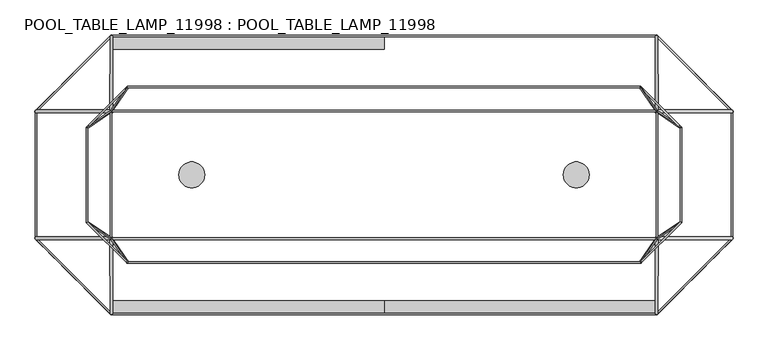
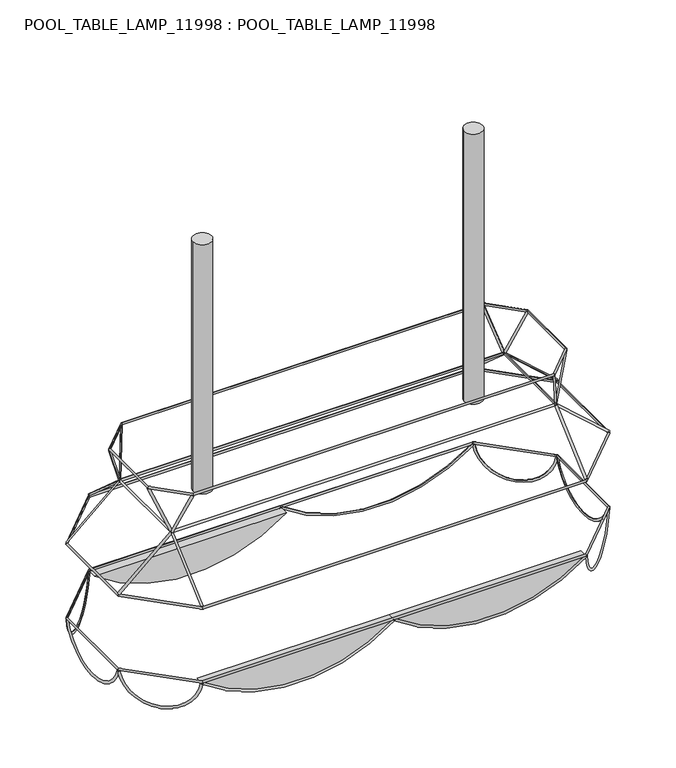
"""IFC4 building model written with IfcOpenShell, lengths in millimetres: proxy geometry, POOL_TABLE_LAMP_11998 : POOL_TABLE_LAMP_11998."""

from ifc_helpers import new_model, si_unit, point, frame, frame_2d, origin, origin_2d, place, context, project, spatial, polyline, circle_curve, ellipse_curve, trimmed, segment, composite_curve, outline, extrude, source, transform, mapped, element, save
from ifc_brep_helpers import plane_surface, cylinder_surface, revolved_surface, advanced_brep


def pool_table_lamp_11998_pool_table_lamp_11998_82cd1bbc(model_context):
    return source(origin(), model_context, "Body", "SolidModel", [
        extrude(outline(composite_curve([segment(trimmed(circle_curve(frame_2d((-308.8341807, 246.5034627)), 25.4), [point((-283.4341807, 246.5034627))], [point((-334.2341807, 246.5034627))], False, "CARTESIAN"), True, "CONTINUOUS"), segment(trimmed(circle_curve(frame_2d((-308.8341807, 246.5034627)), 25.4), [point((-334.2341807, 246.5034627))], [point((-283.4341807, 246.5034627))], False, "CARTESIAN"), True, "CONTINUOUS")], self_intersect=False)), frame((0.0, 0.0, 2030.2376392), z_axis=(0.0, 0.0, 1.0), x_axis=(1.0, 0.0, 0.0)), (0.0, 0.0, 1.0), 792.7919161),
        extrude(outline(composite_curve([segment(trimmed(circle_curve(frame_2d((-1061.7579936, 246.5034627)), 25.4), [point((-1087.1579936, 246.5034627))], [point((-1036.3579936, 246.5034627))], False, "CARTESIAN"), True, "CONTINUOUS"), segment(trimmed(circle_curve(frame_2d((-1061.7579936, 246.5034627)), 25.4), [point((-1036.3579936, 246.5034627))], [point((-1087.1579936, 246.5034627))], False, "CARTESIAN"), True, "CONTINUOUS")], self_intersect=False)), frame((0.0, 0.0, 2030.2376392), z_axis=(0.0, 0.0, 1.0), x_axis=(1.0, 0.0, 0.0)), (0.0, 0.0, 1.0), 731.5822221),
        extrude(outline(composite_curve([segment(polyline([(0.0, -3.175), (0.0, 3.175)]), True, "CONTINUOUS"), segment(trimmed(circle_curve(origin_2d(), 3.175), [point((0.0, 3.175))], [point((0.0, -3.175))], False, "CARTESIAN"), True, "CONTINUOUS")], self_intersect=False)), frame((-1218.1975115, 370.1790475, 2030.2376392), z_axis=(-0.3368565795297006, -0.2287745741588877, 0.9133399361935128), x_axis=(-0.7046441830524278, 0.7046441830524578, -0.08338555378907853)), (0.0, 0.0, 1.0), 138.9524053),
        extrude(outline(composite_curve([segment(polyline([(0.0, -3.175), (0.0, 3.1750001)]), True, "CONTINUOUS"), segment(trimmed(circle_curve(origin_2d(), 3.175), [point((0.0, 3.1750001))], [point((0.0, -3.175))], False, "CARTESIAN"), True, "CONTINUOUS")], self_intersect=False)), frame((-1218.1975115, 122.827878, 2030.2376392), z_axis=(-0.33685657952969905, 0.22877457415888985, 0.9133399361935128), x_axis=(-0.7046441830524323, -0.7046441830524531, -0.08338555378907848)), (0.0, 0.0, 1.0), 138.9524053),
        extrude(outline(composite_curve([segment(polyline([(0.0, -3.1750001), (0.0, 3.175)]), True, "CONTINUOUS"), segment(trimmed(circle_curve(origin_2d(), 3.175), [point((0.0, 3.175))], [point((0.0, -3.1750001))], False, "CARTESIAN"), True, "CONTINUOUS")], self_intersect=False)), frame((-152.3946628, 122.827878, 2030.2376392), z_axis=(0.33685657952969905, 0.22877457415888985, 0.9133399361935128), x_axis=(0.7046441830524323, -0.7046441830524531, -0.08338555378907847)), (0.0, 0.0, 1.0), 138.9524053),
        extrude(outline(composite_curve([segment(polyline([(0.0, -3.175), (0.0, 3.175)]), True, "CONTINUOUS"), segment(trimmed(circle_curve(origin_2d(), 3.175), [point((0.0, 3.175))], [point((0.0, -3.175))], False, "CARTESIAN"), True, "CONTINUOUS")], self_intersect=False)), frame((-152.3946628, 370.1790475, 2030.2376392), z_axis=(0.33685657952969744, -0.22877457415889219, 0.9133399361935128), x_axis=(0.704644183052437, 0.7046441830524486, -0.08338555378907836)), (0.0, 0.0, 1.0), 138.9524053),
        extrude(outline(composite_curve([segment(polyline([(0.0, -3.1749999), (0.0, 3.175)]), True, "CONTINUOUS"), segment(trimmed(circle_curve(origin_2d(), 3.175), [point((0.0, 3.175))], [point((0.0, -3.1749999))], False, "CARTESIAN"), True, "CONTINUOUS")], self_intersect=False)), frame((-152.2155087, 369.9998934, 2030.2376392), z_axis=(-0.22877457415889185, 0.33685657952969766, 0.9133399361935128), x_axis=(0.7046441830524492, 0.7046441830524363, -0.0833855537890783)), (0.0, 0.0, 1.0), 138.9524053),
        extrude(outline(composite_curve([segment(polyline([(0.0, -3.175), (0.0, 3.175)]), True, "CONTINUOUS"), segment(trimmed(circle_curve(origin_2d(), 3.175), [point((0.0, 3.175))], [point((0.0, -3.175))], False, "CARTESIAN"), True, "CONTINUOUS")], self_intersect=False)), frame((-152.2155087, 123.007032, 2030.2376392), z_axis=(-0.22877457415889405, -0.3368565795296962, 0.9133399361935128), x_axis=(0.7046441830524446, -0.704644183052441, -0.08338555378907837)), (0.0, 0.0, 1.0), 138.9524053),
        extrude(outline(composite_curve([segment(polyline([(0.0, -3.1750001), (0.0, 3.175)]), True, "CONTINUOUS"), segment(trimmed(circle_curve(origin_2d(), 3.175), [point((0.0, 3.175))], [point((0.0, -3.1750001))], False, "CARTESIAN"), True, "CONTINUOUS")], self_intersect=False)), frame((-1218.3766655, 123.007032, 2030.2376392), z_axis=(0.22877457415889405, -0.3368565795296962, 0.9133399361935128), x_axis=(-0.7046441830524446, -0.704644183052441, -0.08338555378907837)), (0.0, 0.0, 1.0), 138.9524053),
        extrude(outline(composite_curve([segment(polyline([(0.0, -3.175), (1e-07, 3.175)]), True, "CONTINUOUS"), segment(trimmed(circle_curve(origin_2d(), 3.175), [point((1e-07, 3.175))], [point((0.0, -3.175))], False, "CARTESIAN"), True, "CONTINUOUS")], self_intersect=False)), frame((-1218.3766655, 369.9998934, 2030.2376392), z_axis=(0.22877457415889615, 0.33685657952969483, 0.9133399361935128), x_axis=(-0.70464418305244, 0.7046441830524455, -0.0833855537890785)), (0.0, 0.0, 1.0), 138.9524053),
        advanced_brep(
        [(-105.6341807, 338.43682, 2162.175), (-184.0042861, 416.8069254, 2162.175), (-184.0042861, 416.8069254, 2155.825), (-105.6341807, 338.43682, 2155.825), (-1186.5878882, 416.8069254, 2162.175), (-1186.5878882, 416.8069254, 2155.825), (-1264.9579936, 338.43682, 2162.175), (-1264.9579936, 338.43682, 2155.825), (-1264.9579936, 154.5701054, 2162.175), (-1264.9579936, 154.5701054, 2155.825), (-1186.5878882, 76.2, 2162.175), (-1186.5878882, 76.2, 2155.825), (-184.0042861, 76.2, 2162.175), (-184.0042861, 76.2, 2155.825), (-105.6341807, 154.5701054, 2162.175), (-105.6341807, 154.5701054, 2155.825)],
        [
            (0, 1),
            (1, 2),
            (2, 3),
            (3, 0),
            (0, 3, ellipse_curve(frame((-105.6341807, 338.43682, 2159.0), z_axis=(-0.38268343236509084, 0.9238795325112865, 0.0), x_axis=(0.923879532511286, 0.38268343236509184, 0.0)), 3.4365952, 3.175)),
            (2, 1, ellipse_curve(frame((-184.0042861, 416.8069254, 2159.0), z_axis=(0.9238795325112863, -0.382683432365091, 0.0), x_axis=(-0.3826834323650911, -0.9238795325112862, 0.0)), 3.4365952, 3.175)),
            (1, 4),
            (4, 5),
            (5, 2),
            (5, 4, ellipse_curve(frame((-1186.5878882, 416.8069254, 2159.0), z_axis=(0.9238795325112887, 0.38268343236508495, 0.0), x_axis=(0.38268343236508523, -0.9238795325112888, 0.0)), 3.4365952, 3.175)),
            (4, 6),
            (6, 7),
            (7, 5),
            (7, 6, ellipse_curve(frame((-1264.9579936, 338.43682, 2159.0), z_axis=(0.38268343236509156, 0.9238795325112859, 0.0), x_axis=(0.9238795325112862, -0.3826834323650906, 0.0)), 3.4365952, 3.175)),
            (6, 8),
            (8, 9),
            (9, 7),
            (9, 8, ellipse_curve(frame((-1264.9579936, 154.5701054, 2159.0), z_axis=(-0.38268343236508867, 0.9238795325112872, 0.0), x_axis=(0.9238795325112872, 0.38268343236508895, 0.0)), 3.4365952, 3.175)),
            (8, 10),
            (10, 11),
            (11, 9),
            (11, 10, ellipse_curve(frame((-1186.5878882, 76.2, 2159.0), z_axis=(-0.9238795325112863, 0.38268343236509084, 0.0), x_axis=(0.38268343236509084, 0.9238795325112864, 0.0)), 3.4365952, 3.175)),
            (10, 12),
            (12, 13),
            (13, 11),
            (13, 12, ellipse_curve(frame((-184.0042861, 76.2, 2159.0), z_axis=(-0.9238795325112887, -0.38268343236508484, 0.0), x_axis=(-0.3826834323650852, 0.9238795325112886, 0.0)), 3.4365952, 3.175)),
            (12, 14),
            (14, 15),
            (15, 13),
            (15, 14, ellipse_curve(frame((-105.6341807, 154.5701054, 2159.0), z_axis=(-0.38268343236509555, -0.9238795325112844, 0.0), x_axis=(-0.9238795325112842, 0.38268343236509583, 0.0)), 3.4365952, 3.175)),
            (14, 0),
            (3, 15),
        ],
        [
            plane_surface(frame((-105.6341807, 338.43682, 2159.0), z_axis=(-0.7071067811865449, -0.7071067811865501, 0.0), x_axis=(-0.7071067811865501, 0.7071067811865449, 0.0))),
            cylinder_surface(frame((-105.6341807, 338.43682, 2159.0), z_axis=(0.7071067811865503, -0.7071067811865448, 0.0), x_axis=(-0.7071067811865448, -0.7071067811865503, 0.0)), 3.175),
            plane_surface(frame((-184.0042861, 416.8069254, 2159.0), z_axis=(0.0, -1.0, 0.0), x_axis=(-1.0, 0.0, 0.0))),
            cylinder_surface(frame((-184.0042861, 416.8069254, 2159.0), z_axis=(1.0, 0.0, 0.0), x_axis=(0.0, -1.0, 0.0)), 3.175),
            plane_surface(frame((-1186.5878882, 416.8069254, 2159.0), z_axis=(0.7071067811865451, -0.70710678118655, 0.0), x_axis=(-0.70710678118655, -0.7071067811865451, 0.0))),
            cylinder_surface(frame((-1186.5878882, 416.8069254, 2159.0), z_axis=(0.7071067811865503, 0.7071067811865448, 0.0), x_axis=(0.7071067811865448, -0.7071067811865503, 0.0)), 3.175),
            plane_surface(frame((-1264.9579936, 338.43682, 2159.0), z_axis=(1.0, 0.0, 0.0), x_axis=(0.0, -1.0, 0.0))),
            cylinder_surface(frame((-1264.9579936, 338.43682, 2159.0), z_axis=(0.0, 1.0, 0.0), x_axis=(1.0, 0.0, 0.0)), 3.175),
            plane_surface(frame((-1264.9579936, 154.5701054, 2159.0), z_axis=(0.7071067811865496, 0.7071067811865456, 0.0), x_axis=(0.7071067811865456, -0.7071067811865496, 0.0))),
            cylinder_surface(frame((-1264.9579936, 154.5701054, 2159.0), z_axis=(-0.7071067811865459, 0.7071067811865491, 0.0), x_axis=(0.7071067811865491, 0.7071067811865459, 0.0)), 3.175),
            plane_surface(frame((-1186.5878882, 76.2, 2159.0), z_axis=(0.0, 1.0, 0.0), x_axis=(1.0, 0.0, 0.0))),
            cylinder_surface(frame((-1186.5878882, 76.2, 2159.0), z_axis=(-1.0, 0.0, 0.0), x_axis=(0.0, 1.0, 0.0)), 3.175),
            plane_surface(frame((-184.0042861, 76.2, 2159.0), z_axis=(-0.70710678118654, 0.7071067811865551, 0.0), x_axis=(0.7071067811865551, 0.70710678118654, 0.0))),
            cylinder_surface(frame((-184.0042861, 76.2, 2159.0), z_axis=(-0.7071067811865551, -0.70710678118654, 0.0), x_axis=(-0.70710678118654, 0.7071067811865551, 0.0)), 3.175),
            plane_surface(frame((-105.6341807, 154.5701054, 2159.0), z_axis=(-1.0, 0.0, 0.0), x_axis=(0.0, 1.0, 0.0))),
            cylinder_surface(frame((-105.6341807, 154.5701054, 2159.0), z_axis=(0.0, -1.0, 0.0), x_axis=(-1.0, 0.0, 0.0)), 3.175),
        ],
        [
            (0, [[1, 2, 3, 4]]),
            (1, [[5, -3, 6, -1]]),
            (2, [[-2, 7, 8, 9]]),
            (3, [[-6, -9, 10, -7]]),
            (4, [[-8, 11, 12, 13]]),
            (5, [[-10, -13, 14, -11]]),
            (6, [[-12, 15, 16, 17]]),
            (7, [[-14, -17, 18, -15]]),
            (8, [[-16, 19, 20, 21]]),
            (9, [[-18, -21, 22, -19]]),
            (10, [[-20, 23, 24, 25]]),
            (11, [[-22, -25, 26, -23]]),
            (12, [[-24, 27, 28, 29]]),
            (13, [[-26, -29, 30, -27]]),
            (14, [[-28, 31, -4, 32]]),
            (15, [[-30, -32, -5, -31]]),
        ],
    ),
        advanced_brep(
        [(-1218.3766655, 123.007032, 2028.825), (-1218.3766655, 123.007032, 2035.175), (-1218.3766655, 369.9998934, 2035.175), (-1218.3766655, 369.9998934, 2028.825), (-152.2155087, 369.9998934, 2035.175), (-152.2155087, 369.9998934, 2028.825), (-152.2155087, 123.007032, 2035.175), (-152.2155087, 123.007032, 2028.825)],
        [
            (0, 1, ellipse_curve(frame((-1218.3766655, 123.007032, 2032.0), z_axis=(-0.707106781186548, 0.707106781186547, 0.0), x_axis=(-0.707106781186547, -0.7071067811865479, 0.0)), 4.4901281, 3.175)),
            (1, 2),
            (2, 3, ellipse_curve(frame((-1218.3766655, 369.9998934, 2032.0), z_axis=(-0.7071067811865492, -0.7071067811865457, 0.0), x_axis=(0.7071067811865456, -0.7071067811865493, 0.0)), 4.4901281, 3.175)),
            (3, 0),
            (3, 2),
            (1, 0),
            (2, 4),
            (4, 5, ellipse_curve(frame((-152.2155087, 369.9998934, 2032.0), z_axis=(-0.7071067811865446, 0.7071067811865506, 0.0), x_axis=(-0.7071067811865505, -0.7071067811865446, 0.0)), 4.4901281, 3.175)),
            (5, 3),
            (5, 4),
            (4, 6),
            (6, 7, ellipse_curve(frame((-152.2155087, 123.007032, 2032.0), z_axis=(0.7071067811865482, 0.7071067811865468, 0.0), x_axis=(-0.7071067811865468, 0.7071067811865482, 0.0)), 4.4901281, 3.175)),
            (7, 5),
            (7, 6),
            (6, 1),
            (0, 7),
        ],
        [
            cylinder_surface(frame((-1218.3766655, 123.007032, 2032.0), z_axis=(0.0, -1.0, 0.0), x_axis=(-1.0, 0.0, 0.0)), 3.175),
            plane_surface(frame((-1218.3766655, 123.007032, 2032.0), z_axis=(1.0, 0.0, 0.0), x_axis=(0.0, 1.0, 0.0))),
            cylinder_surface(frame((-1218.3766655, 369.9998934, 2032.0), z_axis=(-1.0, 0.0, 0.0), x_axis=(0.0, 1.0, 0.0)), 3.175),
            plane_surface(frame((-1218.3766655, 369.9998934, 2032.0), z_axis=(0.0, -1.0, 0.0), x_axis=(1.0, 0.0, 0.0))),
            cylinder_surface(frame((-152.2155087, 369.9998934, 2032.0), z_axis=(0.0, 1.0, 0.0), x_axis=(1.0, 0.0, 0.0)), 3.175),
            plane_surface(frame((-152.2155087, 369.9998934, 2032.0), z_axis=(-1.0, 0.0, 0.0), x_axis=(0.0, -1.0, 0.0))),
            cylinder_surface(frame((-152.2155087, 123.007032, 2032.0), z_axis=(1.0, 0.0, 0.0), x_axis=(0.0, -1.0, 0.0)), 3.175),
            plane_surface(frame((-152.2155087, 123.007032, 2032.0), z_axis=(0.0, 1.0, 0.0), x_axis=(-1.0, 0.0, 0.0))),
        ],
        [
            (0, [[1, 2, 3, 4]]),
            (1, [[-4, 5, -2, 6]]),
            (2, [[-3, 7, 8, 9]]),
            (3, [[-5, -9, 10, -7]]),
            (4, [[-8, 11, 12, 13]]),
            (5, [[-10, -13, 14, -11]]),
            (6, [[-12, 15, -1, 16]]),
            (7, [[-14, -16, -6, -15]]),
        ],
    ),
        advanced_brep(
        [(-1365.4872204, 366.9890164, 1677.4075935), (-1365.4872204, 373.0107705, 1675.3924065), (-1365.4872204, 119.996155, 1675.3924065), (-1365.4872204, 126.017909, 1677.4075935)],
        [
            (0, 1),
            (1, 0, circle_curve(frame((-1365.4872204, 369.9998934, 1676.4), z_axis=(0.0, 0.3173522867463232, 0.9483077169868858), x_axis=(0.0, 0.9483077169868858, -0.3173522867463232)), 3.175)),
            (2, 3),
            (3, 2, circle_curve(frame((-1365.4872204, 123.007032, 1676.4), z_axis=(0.0, -0.3173522867463063, 0.9483077169868914), x_axis=(0.0, -0.9483077169868914, -0.3173522867463063)), 3.175)),
            (3, 0, circle_curve(frame((-1365.4872204, 246.5034627, 1717.728225), z_axis=(1.0, 0.0, 0.0), x_axis=(0.0, 0.9483077169868859, -0.317352286746323)), 127.053225)),
            (1, 2, circle_curve(frame((-1365.4872204, 246.5034627, 1717.728225), z_axis=(-1.0, 0.0, 0.0), x_axis=(0.0, 0.9483077169868859, -0.317352286746323)), 133.403225)),
        ],
        [
            plane_surface(frame((-1365.4872204, 369.9998934, 1676.4), z_axis=(0.0, 0.317352286746323, 0.9483077169868859), x_axis=(-1.0, 0.0, 0.0))),
            plane_surface(frame((-1365.4872204, 123.007032, 1676.4), z_axis=(0.0, -0.31735228674630656, 0.9483077169868913), x_axis=(-1.0, 0.0, 0.0))),
            revolved_surface(trimmed(ellipse_curve(frame((-1365.4872204, 369.9998934, 1676.4), z_axis=(0.0, 0.3173522867463232, 0.9483077169868858), x_axis=(0.0, 0.9483077169868858, -0.3173522867463232)), 3.175, 3.175), [point((-1365.4872204, 373.0107705, 1675.3924065))], [point((-1365.4872204, 366.9890164, 1677.4075935))], True, "CARTESIAN"), (-1365.4872204, 246.5034627, 1717.728225), (-1.0, 0.0, 0.0)),
            plane_surface(frame((-1365.4872204, 246.5034627, 1717.728225), z_axis=(1.0, 0.0, 0.0), x_axis=(0.0, 0.9483077169868859, -0.317352286746323))),
        ],
        [
            (0, [[1, 2]]),
            (1, [[3, 4]]),
            (2, [[5, -2, 6, -4]]),
            (3, [[-6, -1, -5, -3]]),
        ],
    ),
        advanced_brep(
        [(-5.1049539, 373.0107705, 1675.3924065), (-5.1049539, 366.9890164, 1677.4075935), (-5.1049539, 126.017909, 1677.4075935), (-5.1049539, 119.996155, 1675.3924065)],
        [
            (0, 1),
            (1, 0, circle_curve(frame((-5.1049539, 369.9998934, 1676.4), z_axis=(0.0, 0.3173522867463232, 0.9483077169868858), x_axis=(0.0, 0.9483077169868858, -0.3173522867463232)), 3.175)),
            (2, 3),
            (3, 2, circle_curve(frame((-5.1049539, 123.007032, 1676.4), z_axis=(0.0, -0.3173522867463063, 0.9483077169868914), x_axis=(0.0, -0.9483077169868914, -0.3173522867463063)), 3.175)),
            (3, 0, circle_curve(frame((-5.1049539, 246.5034627, 1717.728225), z_axis=(1.0, 0.0, 0.0), x_axis=(0.0, 0.9483077169868859, -0.317352286746323)), 133.403225)),
            (1, 2, circle_curve(frame((-5.1049539, 246.5034627, 1717.728225), z_axis=(-1.0, 0.0, 0.0), x_axis=(0.0, 0.9483077169868859, -0.317352286746323)), 127.053225)),
        ],
        [
            plane_surface(frame((-5.1049539, 369.9998934, 1676.4), z_axis=(0.0, 0.317352286746323, 0.9483077169868859), x_axis=(1.0, 0.0, 0.0))),
            plane_surface(frame((-5.1049539, 123.007032, 1676.4), z_axis=(0.0, -0.31735228674630656, 0.9483077169868913), x_axis=(1.0, 0.0, 0.0))),
            revolved_surface(trimmed(ellipse_curve(frame((-5.1049539, 369.9998934, 1676.4), z_axis=(0.0, 0.3173522867463232, 0.9483077169868858), x_axis=(0.0, 0.9483077169868858, -0.3173522867463232)), 3.175, 3.175), [point((-5.1049539, 366.9890164, 1677.4075935))], [point((-5.1049539, 373.0107705, 1675.3924065))], True, "CARTESIAN"), (-5.1049539, 246.5034627, 1717.728225), (-1.0, 0.0, 0.0)),
            plane_surface(frame((-5.1049539, 246.5034627, 1717.728225), z_axis=(-1.0, 0.0, 0.0), x_axis=(0.0, 0.9483077169868859, -0.317352286746323))),
        ],
        [
            (0, [[1, 2]]),
            (1, [[3, 4]]),
            (2, [[5, -2, 6, -4]]),
            (3, [[-6, -1, -5, -3]]),
        ],
    ),
        advanced_brep(
        [(-1363.4950625, 120.7891702, 1676.8927506), (-1367.9307861, 125.2248938, 1675.9072494), (-1216.4782253, -26.227667, 1675.9072494), (-1220.9139489, -21.7919434, 1676.8927506)],
        [
            (0, 1),
            (1, 0, circle_curve(frame((-1365.7129243, 123.007032, 1676.4), z_axis=(-0.10974087344321956, 0.1097408734432232, 0.9878835363502307), x_axis=(-0.6985391475757914, 0.6985391475757993, -0.15519703157007309)), 3.175)),
            (2, 3),
            (3, 2, circle_curve(frame((-1218.6960871, -24.0098052, 1676.4), z_axis=(0.10974087344321433, -0.10974087344321463, 0.9878835363502323), x_axis=(0.6985391475757923, -0.6985391475758007, -0.1551970315700634)), 3.175)),
            (3, 0, circle_curve(frame((-1292.2045057, 49.4986134, 1692.7316378), z_axis=(0.7071067811865517, 0.7071067811865435, 0.0), x_axis=(-0.6985391475757914, 0.6985391475757993, -0.1551970315700732)), 102.0566378)),
            (1, 2, circle_curve(frame((-1292.2045057, 49.4986134, 1692.7316378), z_axis=(-0.7071067811865517, -0.7071067811865435, 0.0), x_axis=(-0.6985391475757914, 0.6985391475757993, -0.1551970315700732)), 108.4066378)),
        ],
        [
            plane_surface(frame((-1365.7129243, 123.007032, 1676.4), z_axis=(-0.10974087344321996, 0.10974087344322306, 0.987883536350231), x_axis=(-0.7071067811865518, -0.7071067811865435, 0.0))),
            plane_surface(frame((-1218.6960871, -24.0098052, 1676.4), z_axis=(0.10974087344321468, -0.10974087344321405, 0.9878835363502325), x_axis=(-0.7071067811865517, -0.7071067811865436, 0.0))),
            revolved_surface(trimmed(ellipse_curve(frame((-1365.7129243, 123.007032, 1676.4), z_axis=(-0.10974087344321956, 0.1097408734432232, 0.9878835363502307), x_axis=(-0.6985391475757914, 0.6985391475757993, -0.15519703157007309)), 3.175, 3.175), [point((-1367.9307861, 125.2248938, 1675.9072494))], [point((-1363.4950625, 120.7891702, 1676.8927506))], True, "CARTESIAN"), (-1292.2045057, 49.4986134, 1692.7316378), (-0.7071067811865517, -0.7071067811865435, 0.0)),
            plane_surface(frame((-1292.2045057, 49.4986134, 1692.7316378), z_axis=(0.7071067811865517, 0.7071067811865435, 0.0), x_axis=(-0.6985391475757915, 0.6985391475757994, -0.15519703157007322))),
        ],
        [
            (0, [[1, 2]]),
            (1, [[3, 4]]),
            (2, [[5, -2, 6, -4]]),
            (3, [[-6, -1, -5, -3]]),
        ],
    ),
        advanced_brep(
        [(-1367.9307861, 367.7820317, 1675.9072494), (-1363.4950625, 372.2177552, 1676.8927506), (-1220.9139489, 514.7988688, 1676.8927506), (-1216.4782253, 519.2345924, 1675.9072494)],
        [
            (0, 1),
            (1, 0, circle_curve(frame((-1365.7129243, 369.9998934, 1676.4), z_axis=(-0.10974087344322034, -0.10974087344322242, 0.987883536350231), x_axis=(-0.6985391475757958, -0.6985391475757948, -0.15519703157007306)), 3.175)),
            (2, 3),
            (3, 2, circle_curve(frame((-1218.6960871, 517.0167306, 1676.4), z_axis=(0.10974087344321516, 0.10974087344321382, 0.9878835363502325), x_axis=(0.6985391475757969, 0.698539147575796, -0.15519703157006345)), 3.175)),
            (3, 0, circle_curve(frame((-1292.2045057, 443.508312, 1692.7316378), z_axis=(-0.7071067811865471, 0.707106781186548, 0.0), x_axis=(-0.6985391475757959, -0.6985391475757947, -0.1551970315700732)), 108.4066378)),
            (1, 2, circle_curve(frame((-1292.2045057, 443.508312, 1692.7316378), z_axis=(0.7071067811865471, -0.707106781186548, 0.0), x_axis=(-0.6985391475757959, -0.6985391475757947, -0.1551970315700732)), 102.0566378)),
        ],
        [
            plane_surface(frame((-1365.7129243, 369.9998934, 1676.4), z_axis=(-0.10974087344322059, -0.10974087344322228, 0.9878835363502307), x_axis=(-0.7071067811865471, 0.7071067811865479, 0.0))),
            plane_surface(frame((-1218.6960871, 517.0167306, 1676.4), z_axis=(0.10974087344321533, 0.10974087344321337, 0.9878835363502325), x_axis=(-0.707106781186547, 0.707106781186548, 0.0))),
            revolved_surface(trimmed(ellipse_curve(frame((-1365.7129243, 369.9998934, 1676.4), z_axis=(-0.10974087344322034, -0.10974087344322242, 0.987883536350231), x_axis=(-0.6985391475757958, -0.6985391475757948, -0.15519703157007306)), 3.175, 3.175), [point((-1363.4950625, 372.2177552, 1676.8927506))], [point((-1367.9307861, 367.7820317, 1675.9072494))], True, "CARTESIAN"), (-1292.2045057, 443.508312, 1692.7316378), (0.7071067811865472, -0.7071067811865481, 0.0)),
            plane_surface(frame((-1292.2045057, 443.508312, 1692.7316378), z_axis=(0.707106781186547, -0.707106781186548, 0.0), x_axis=(-0.698539147575796, -0.6985391475757948, -0.15519703157007322))),
        ],
        [
            (0, [[1, 2]]),
            (1, [[3, 4]]),
            (2, [[5, -2, 6, -4]]),
            (3, [[-6, -1, -5, -3]]),
        ],
    ),
        advanced_brep(
        [(-7.0971118, 372.2177552, 1676.8927506), (-2.6613882, 367.7820317, 1675.9072494), (-154.1139489, 519.2345924, 1675.9072494), (-149.6782253, 514.7988688, 1676.8927506)],
        [
            (0, 1),
            (1, 0, circle_curve(frame((-4.87925, 369.9998934, 1676.4), z_axis=(0.10974087344322034, -0.10974087344322242, 0.987883536350231), x_axis=(0.6985391475757958, -0.6985391475757948, -0.15519703157007306)), 3.175)),
            (2, 3),
            (3, 2, circle_curve(frame((-151.8960871, 517.0167306, 1676.4), z_axis=(-0.10974087344321516, 0.10974087344321382, 0.9878835363502325), x_axis=(-0.6985391475757969, 0.698539147575796, -0.15519703157006345)), 3.175)),
            (3, 0, circle_curve(frame((-78.3876685, 443.508312, 1692.7316378), z_axis=(-0.7071067811865471, -0.707106781186548, 0.0), x_axis=(0.6985391475757959, -0.6985391475757947, -0.1551970315700732)), 102.0566378)),
            (1, 2, circle_curve(frame((-78.3876685, 443.508312, 1692.7316378), z_axis=(0.7071067811865471, 0.707106781186548, 0.0), x_axis=(0.6985391475757959, -0.6985391475757947, -0.1551970315700732)), 108.4066378)),
        ],
        [
            plane_surface(frame((-4.87925, 369.9998934, 1676.4), z_axis=(0.10974087344322059, -0.10974087344322228, 0.9878835363502307), x_axis=(0.7071067811865471, 0.7071067811865479, 0.0))),
            plane_surface(frame((-151.8960871, 517.0167306, 1676.4), z_axis=(-0.10974087344321533, 0.10974087344321337, 0.9878835363502325), x_axis=(0.707106781186547, 0.707106781186548, 0.0))),
            revolved_surface(trimmed(ellipse_curve(frame((-4.87925, 369.9998934, 1676.4), z_axis=(0.10974087344322034, -0.10974087344322242, 0.987883536350231), x_axis=(0.6985391475757958, -0.6985391475757948, -0.15519703157007306)), 3.175, 3.175), [point((-2.6613882, 367.7820317, 1675.9072494))], [point((-7.0971118, 372.2177552, 1676.8927506))], True, "CARTESIAN"), (-78.3876685, 443.508312, 1692.7316378), (0.7071067811865472, 0.7071067811865481, 0.0)),
            plane_surface(frame((-78.3876685, 443.508312, 1692.7316378), z_axis=(-0.707106781186547, -0.707106781186548, 0.0), x_axis=(0.698539147575796, -0.6985391475757948, -0.15519703157007322))),
        ],
        [
            (0, [[1, 2]]),
            (1, [[3, 4]]),
            (2, [[5, -2, 6, -4]]),
            (3, [[-6, -1, -5, -3]]),
        ],
    ),
        advanced_brep(
        [(-2.6613882, 125.2248938, 1675.9072494), (-7.0971118, 120.7891702, 1676.8927506), (-149.6782253, -21.7919434, 1676.8927506), (-154.1139489, -26.227667, 1675.9072494)],
        [
            (0, 1),
            (1, 0, circle_curve(frame((-4.87925, 123.007032, 1676.4), z_axis=(0.10974087344322131, 0.1097408734432216, 0.987883536350231), x_axis=(0.6985391475758004, 0.6985391475757904, -0.15519703157007317)), 3.175)),
            (2, 3),
            (3, 2, circle_curve(frame((-151.8960871, -24.0098052, 1676.4), z_axis=(-0.10974087344321602, -0.10974087344321283, 0.9878835363502325), x_axis=(-0.6985391475758015, -0.6985391475757915, -0.15519703157006334)), 3.175)),
            (3, 0, circle_curve(frame((-78.3876685, 49.4986134, 1692.7316378), z_axis=(0.7071067811865425, -0.7071067811865526, 0.0), x_axis=(0.6985391475758005, 0.6985391475757903, -0.1551970315700732)), 108.4066378)),
            (1, 2, circle_curve(frame((-78.3876685, 49.4986134, 1692.7316378), z_axis=(-0.7071067811865425, 0.7071067811865526, 0.0), x_axis=(0.6985391475758005, 0.6985391475757903, -0.1551970315700732)), 102.0566378)),
        ],
        [
            plane_surface(frame((-4.87925, 123.007032, 1676.4), z_axis=(0.10974087344322135, 0.10974087344322168, 0.9878835363502307), x_axis=(0.7071067811865426, -0.7071067811865526, 0.0))),
            plane_surface(frame((-151.8960871, -24.0098052, 1676.4), z_axis=(-0.10974087344321597, -0.10974087344321265, 0.9878835363502325), x_axis=(0.7071067811865425, -0.7071067811865528, 0.0))),
            revolved_surface(trimmed(ellipse_curve(frame((-4.87925, 123.007032, 1676.4), z_axis=(0.10974087344322131, 0.1097408734432216, 0.987883536350231), x_axis=(0.6985391475758004, 0.6985391475757904, -0.15519703157007317)), 3.175, 3.175), [point((-7.0971118, 120.7891702, 1676.8927506))], [point((-2.6613882, 125.2248938, 1675.9072494))], True, "CARTESIAN"), (-78.3876685, 49.4986134, 1692.7316378), (-0.7071067811865426, 0.7071067811865527, 0.0)),
            plane_surface(frame((-78.3876685, 49.4986134, 1692.7316378), z_axis=(-0.7071067811865425, 0.7071067811865526, 0.0), x_axis=(0.6985391475758005, 0.6985391475757903, -0.1551970315700732))),
        ],
        [
            (0, [[1, 2]]),
            (1, [[3, 4]]),
            (2, [[5, -2, 6, -4]]),
            (3, [[-6, -1, -5, -3]]),
        ],
    ),
        advanced_brep(
        [(-683.3910871, -24.3292268, 1678.94), (-687.2010871, -24.3292268, 1673.86), (-149.9910871, -24.3292268, 1673.86), (-153.8010871, -24.3292268, 1678.94)],
        [
            (0, 1),
            (1, 0, circle_curve(frame((-685.2960871, -24.3292268, 1676.4), z_axis=(-0.7999999999999984, 0.0, 0.6000000000000022), x_axis=(-0.6000000000000022, 0.0, -0.7999999999999984)), 3.175)),
            (2, 3),
            (3, 2, circle_curve(frame((-151.8960871, -24.3292268, 1676.4), z_axis=(0.8000000000000023, 0.0, 0.5999999999999969), x_axis=(0.5999999999999969, 0.0, -0.8000000000000023)), 3.175)),
            (3, 0, circle_curve(frame((-418.5960871, -24.3292268, 2032.0), z_axis=(0.0, 1.0, 0.0), x_axis=(-0.6000000000000022, 0.0, -0.7999999999999984)), 441.325)),
            (1, 2, circle_curve(frame((-418.5960871, -24.3292268, 2032.0), z_axis=(0.0, -1.0, 0.0), x_axis=(-0.6000000000000022, 0.0, -0.7999999999999984)), 447.675)),
        ],
        [
            plane_surface(frame((-685.2960871, -24.3292268, 1676.4), z_axis=(-0.7999999999999984, 0.0, 0.6000000000000022), x_axis=(0.0, -1.0, 0.0))),
            plane_surface(frame((-151.8960871, -24.3292268, 1676.4), z_axis=(0.8000000000000024, 0.0, 0.5999999999999969), x_axis=(0.0, -1.0, 0.0))),
            revolved_surface(trimmed(ellipse_curve(frame((-685.2960871, -24.3292268, 1676.4), z_axis=(-0.7999999999999984, 0.0, 0.6000000000000022), x_axis=(-0.6000000000000022, 0.0, -0.7999999999999984)), 3.175, 3.175), [point((-687.2010871, -24.3292268, 1673.86))], [point((-683.3910871, -24.3292268, 1678.94))], True, "CARTESIAN"), (-418.5960871, -24.3292268, 2032.0), (0.0, -1.0, 0.0)),
            plane_surface(frame((-418.5960871, -24.3292268, 2032.0), z_axis=(0.0, 1.0, 0.0), x_axis=(-0.6000000000000022, 0.0, -0.7999999999999984))),
        ],
        [
            (0, [[1, 2]]),
            (1, [[3, 4]]),
            (2, [[5, -2, 6, -4]]),
            (3, [[-6, -1, -5, -3]]),
        ],
    ),
        advanced_brep(
        [(-687.2010871, 517.3361522, 1673.86), (-683.3910871, 517.3361522, 1678.94), (-153.8010871, 517.3361522, 1678.94), (-149.9910871, 517.3361522, 1673.86)],
        [
            (0, 1),
            (1, 0, circle_curve(frame((-685.2960871, 517.3361522, 1676.4), z_axis=(-0.7999999999999984, 0.0, 0.6000000000000022), x_axis=(-0.6000000000000022, 0.0, -0.7999999999999984)), 3.175)),
            (2, 3),
            (3, 2, circle_curve(frame((-151.8960871, 517.3361522, 1676.4), z_axis=(0.8000000000000023, 0.0, 0.5999999999999969), x_axis=(0.5999999999999969, 0.0, -0.8000000000000023)), 3.175)),
            (3, 0, circle_curve(frame((-418.5960871, 517.3361522, 2032.0), z_axis=(0.0, 1.0, 0.0), x_axis=(-0.6000000000000022, 0.0, -0.7999999999999984)), 447.675)),
            (1, 2, circle_curve(frame((-418.5960871, 517.3361522, 2032.0), z_axis=(0.0, -1.0, 0.0), x_axis=(-0.6000000000000022, 0.0, -0.7999999999999984)), 441.325)),
        ],
        [
            plane_surface(frame((-685.2960871, 517.3361522, 1676.4), z_axis=(-0.7999999999999984, 0.0, 0.6000000000000022), x_axis=(0.0, 1.0, 0.0))),
            plane_surface(frame((-151.8960871, 517.3361522, 1676.4), z_axis=(0.8000000000000024, 0.0, 0.5999999999999969), x_axis=(0.0, 1.0, 0.0))),
            revolved_surface(trimmed(ellipse_curve(frame((-685.2960871, 517.3361522, 1676.4), z_axis=(-0.7999999999999984, 0.0, 0.6000000000000022), x_axis=(-0.6000000000000022, 0.0, -0.7999999999999984)), 3.175, 3.175), [point((-683.3910871, 517.3361522, 1678.94))], [point((-687.2010871, 517.3361522, 1673.86))], True, "CARTESIAN"), (-418.5960871, 517.3361522, 2032.0), (0.0, -1.0, 0.0)),
            plane_surface(frame((-418.5960871, 517.3361522, 2032.0), z_axis=(0.0, -1.0, 0.0), x_axis=(-0.6000000000000022, 0.0, -0.7999999999999984))),
        ],
        [
            (0, [[1, 2]]),
            (1, [[3, 4]]),
            (2, [[5, -2, 6, -4]]),
            (3, [[-6, -1, -5, -3]]),
        ],
    ),
        advanced_brep(
        [(-687.2010871, 517.3361522, 1678.94), (-683.3910871, 517.3361522, 1673.86), (-1220.6010871, 517.3361522, 1673.86), (-1216.7910871, 517.3361522, 1678.94)],
        [
            (0, 1),
            (1, 0, circle_curve(frame((-685.2960871, 517.3361522, 1676.4), z_axis=(0.7999999999999984, 0.0, 0.6000000000000022), x_axis=(0.6000000000000022, 0.0, -0.7999999999999984)), 3.175)),
            (2, 3),
            (3, 2, circle_curve(frame((-1218.6960871, 517.3361522, 1676.4), z_axis=(-0.8000000000000023, 0.0, 0.5999999999999969), x_axis=(-0.5999999999999969, 0.0, -0.8000000000000023)), 3.175)),
            (3, 0, circle_curve(frame((-951.9960871, 517.3361522, 2032.0), z_axis=(0.0, -1.0, 0.0), x_axis=(0.6000000000000022, 0.0, -0.7999999999999984)), 441.325)),
            (1, 2, circle_curve(frame((-951.9960871, 517.3361522, 2032.0), z_axis=(0.0, 1.0, 0.0), x_axis=(0.6000000000000022, 0.0, -0.7999999999999984)), 447.675)),
        ],
        [
            plane_surface(frame((-685.2960871, 517.3361522, 1676.4), z_axis=(0.7999999999999984, 0.0, 0.6000000000000022), x_axis=(0.0, 1.0, 0.0))),
            plane_surface(frame((-1218.6960871, 517.3361522, 1676.4), z_axis=(-0.8000000000000024, 0.0, 0.5999999999999969), x_axis=(0.0, 1.0, 0.0))),
            revolved_surface(trimmed(ellipse_curve(frame((-685.2960871, 517.3361522, 1676.4), z_axis=(0.7999999999999984, 0.0, 0.6000000000000022), x_axis=(0.6000000000000022, 0.0, -0.7999999999999984)), 3.175, 3.175), [point((-683.3910871, 517.3361522, 1673.86))], [point((-687.2010871, 517.3361522, 1678.94))], True, "CARTESIAN"), (-951.9960871, 517.3361522, 2032.0), (0.0, 1.0, 0.0)),
            plane_surface(frame((-951.9960871, 517.3361522, 2032.0), z_axis=(0.0, -1.0, 0.0), x_axis=(0.6000000000000022, 0.0, -0.7999999999999984))),
        ],
        [
            (0, [[1, 2]]),
            (1, [[3, 4]]),
            (2, [[5, -2, 6, -4]]),
            (3, [[-6, -1, -5, -3]]),
        ],
    ),
        advanced_brep(
        [(-683.3910871, -24.3292268, 1673.86), (-687.2010871, -24.3292268, 1678.94), (-1216.7910871, -24.3292268, 1678.94), (-1220.6010871, -24.3292268, 1673.86)],
        [
            (0, 1),
            (1, 0, circle_curve(frame((-685.2960871, -24.3292268, 1676.4), z_axis=(0.7999999999999984, 0.0, 0.6000000000000022), x_axis=(0.6000000000000022, 0.0, -0.7999999999999984)), 3.175)),
            (2, 3),
            (3, 2, circle_curve(frame((-1218.6960871, -24.3292268, 1676.4), z_axis=(-0.8000000000000023, 0.0, 0.5999999999999969), x_axis=(-0.5999999999999969, 0.0, -0.8000000000000023)), 3.175)),
            (3, 0, circle_curve(frame((-951.9960871, -24.3292268, 2032.0), z_axis=(0.0, -1.0, 0.0), x_axis=(0.6000000000000022, 0.0, -0.7999999999999984)), 447.675)),
            (1, 2, circle_curve(frame((-951.9960871, -24.3292268, 2032.0), z_axis=(0.0, 1.0, 0.0), x_axis=(0.6000000000000022, 0.0, -0.7999999999999984)), 441.325)),
        ],
        [
            plane_surface(frame((-685.2960871, -24.3292268, 1676.4), z_axis=(0.7999999999999984, 0.0, 0.6000000000000022), x_axis=(0.0, -1.0, 0.0))),
            plane_surface(frame((-1218.6960871, -24.3292268, 1676.4), z_axis=(-0.8000000000000024, 0.0, 0.5999999999999969), x_axis=(0.0, -1.0, 0.0))),
            revolved_surface(trimmed(ellipse_curve(frame((-685.2960871, -24.3292268, 1676.4), z_axis=(0.7999999999999984, 0.0, 0.6000000000000022), x_axis=(0.6000000000000022, 0.0, -0.7999999999999984)), 3.175, 3.175), [point((-687.2010871, -24.3292268, 1678.94))], [point((-683.3910871, -24.3292268, 1673.86))], True, "CARTESIAN"), (-951.9960871, -24.3292268, 2032.0), (0.0, 1.0, 0.0)),
            plane_surface(frame((-951.9960871, -24.3292268, 2032.0), z_axis=(0.0, 1.0, 0.0), x_axis=(0.6000000000000022, 0.0, -0.7999999999999984))),
        ],
        [
            (0, [[1, 2]]),
            (1, [[3, 4]]),
            (2, [[5, -2, 6, -4]]),
            (3, [[-6, -1, -5, -3]]),
        ],
    ),
        extrude(outline(composite_curve([segment(polyline([(1.0116489, -3.3404831), (1.0116488, 3.0095169)]), True, "CONTINUOUS"), segment(trimmed(circle_curve(frame_2d((1.0116488, -0.1654831)), 3.175), [point((1.0116488, 3.0095169))], [point((1.0116489, -3.3404831))], False, "CARTESIAN"), True, "CONTINUOUS")], self_intersect=False)), frame((-1365.4872204, 122.7813281, 1900.5601186), z_axis=(0.7489760011034178, 0.0011491140369261907, 0.6625961283527572), x_axis=(-0.5520187561669342, -0.5520187561669319, 0.6249404657083941)), (0.0, 0.0, 1.0), 196.415579),
        extrude(outline(composite_curve([segment(trimmed(circle_curve(frame_2d((0.547441, -0.8666755)), 3.175), [point((3.4702869, 0.3733237))], [point((-2.3754047, -2.1066746))], False, "CARTESIAN"), True, "CONTINUOUS"), segment(polyline([(-2.3754047, -2.1066746), (3.4702869, 0.3733237)]), True, "CONTINUOUS")], self_intersect=False)), frame((-1219.5743544, 516.2539214, 1900.5601186), z_axis=(-0.0011491140369209727, -0.7489760011034178, 0.6625961283527572), x_axis=(-0.5520177425656377, 0.5529694008127184, 0.6241003554377779)), (0.0, 0.0, 1.0), 196.415579),
        extrude(outline(composite_curve([segment(polyline([(3.4702869, -0.3733237), (-2.3754046, 2.1066745)]), True, "CONTINUOUS"), segment(trimmed(circle_curve(frame_2d((0.5474411, 0.8666754)), 3.175), [point((-2.3754046, 2.1066745))], [point((3.4702869, -0.3733237))], False, "CARTESIAN"), True, "CONTINUOUS")], self_intersect=False)), frame((-151.0178199, 516.2539214, 1900.5601186), z_axis=(0.0011491140369209727, -0.7489760011034178, 0.6625961283527572), x_axis=(0.5520177425656377, 0.5529694008127184, 0.6241003554377779)), (0.0, 0.0, 1.0), 196.415579),
        extrude(outline(composite_curve([segment(trimmed(circle_curve(frame_2d((0.5474411, -0.8666754)), 3.175), [point((3.4702869, 0.3733237))], [point((-2.3754046, -2.1066745))], False, "CARTESIAN"), True, "CONTINUOUS"), segment(polyline([(-2.3754046, -2.1066745), (3.4702869, 0.3733237)]), True, "CONTINUOUS")], self_intersect=False)), frame((-151.0178199, -23.246996, 1900.5601186), z_axis=(0.00114911403692583, 0.7489760011034178, 0.662596128352757), x_axis=(0.5520177425656341, -0.552969400812722, 0.6241003554377779)), (0.0, 0.0, 1.0), 196.415579),
        extrude(outline(composite_curve([segment(polyline([(3.4702869, -0.3733237), (-2.3754047, 2.1066746)]), True, "CONTINUOUS"), segment(trimmed(circle_curve(frame_2d((0.547441, 0.8666755)), 3.175), [point((-2.3754047, 2.1066746))], [point((3.4702869, -0.3733237))], False, "CARTESIAN"), True, "CONTINUOUS")], self_intersect=False)), frame((-1219.5743544, -23.246996, 1900.5601186), z_axis=(-0.00114911403692583, 0.7489760011034178, 0.662596128352757), x_axis=(-0.5520177425656341, -0.552969400812722, 0.6241003554377779)), (0.0, 0.0, 1.0), 196.415579),
        extrude(outline(composite_curve([segment(trimmed(circle_curve(frame_2d((1.0116488, 0.1654831)), 3.175), [point((1.0116489, 3.3404831))], [point((1.0116488, -3.0095169))], False, "CARTESIAN"), True, "CONTINUOUS"), segment(polyline([(1.0116488, -3.0095169), (1.0116489, 3.3404831)]), True, "CONTINUOUS")], self_intersect=False)), frame((-1365.4872204, 370.2255973, 1900.5601186), z_axis=(0.7489760011034177, -0.001149114036930965, 0.6625961283527573), x_axis=(-0.5520187561669306, 0.5520187561669353, 0.624940465708394)), (0.0, 0.0, 1.0), 196.415579),
        extrude(outline(composite_curve([segment(polyline([(1.0116489, -3.3404831), (1.0116488, 3.0095169)]), True, "CONTINUOUS"), segment(trimmed(circle_curve(frame_2d((1.0116488, -0.1654831)), 3.175), [point((1.0116488, 3.0095169))], [point((1.0116489, -3.3404831))], False, "CARTESIAN"), True, "CONTINUOUS")], self_intersect=False)), frame((-5.1049539, 370.2255973, 1900.5601186), z_axis=(-0.7489760011034177, -0.001149114036930965, 0.6625961283527573), x_axis=(0.5520187561669306, 0.5520187561669353, 0.624940465708394)), (0.0, 0.0, 1.0), 196.415579),
        extrude(outline(composite_curve([segment(trimmed(circle_curve(frame_2d((1.0116488, 0.1654831)), 3.175), [point((1.0116489, 3.3404831))], [point((1.0116488, -3.0095169))], False, "CARTESIAN"), True, "CONTINUOUS"), segment(polyline([(1.0116488, -3.0095169), (1.0116489, 3.3404831)]), True, "CONTINUOUS")], self_intersect=False)), frame((-5.1049539, 122.7813281, 1900.5601186), z_axis=(-0.7489760011034177, 0.001149114036935961, 0.6625961283527574), x_axis=(0.5520187561669272, -0.5520187561669389, 0.6249404657083941)), (0.0, 0.0, 1.0), 196.415579),
        advanced_brep(
        [(-152.2155087, -24.3292268, 1894.2101186), (-152.2155087, -24.3292268, 1900.5601186), (-5.1049539, 122.7813281, 1900.5601186), (-5.1049539, 122.7813281, 1894.2101186), (-5.1049539, 370.2255973, 1900.5601186), (-5.1049539, 370.2255973, 1894.2101186), (-152.2155087, 517.3361522, 1900.5601186), (-152.2155087, 517.3361522, 1894.2101186), (-1218.3766655, 517.3361522, 1900.5601186), (-1218.3766655, 517.3361522, 1894.2101186), (-1365.4872204, 370.2255973, 1900.5601186), (-1365.4872204, 370.2255973, 1894.2101186), (-1365.4872204, 122.7813281, 1900.5601186), (-1365.4872204, 122.7813281, 1894.2101186), (-1218.3766655, -24.3292268, 1900.5601186), (-1218.3766655, -24.3292268, 1894.2101186)],
        [
            (0, 1),
            (1, 2),
            (2, 3),
            (3, 0),
            (1, 0, ellipse_curve(frame((-152.2155087, -24.3292268, 1897.3851186), z_axis=(0.9238795325112887, 0.3826834323650849, 0.0), x_axis=(0.38268343236508473, -0.9238795325112887, 0.0)), 3.4365952, 3.175)),
            (3, 2, ellipse_curve(frame((-5.1049539, 122.7813281, 1897.3851186), z_axis=(-0.3826834323650956, -0.9238795325112844, 0.0), x_axis=(-0.9238795325112843, 0.38268343236509583, 0.0)), 3.4365952, 3.175)),
            (2, 4),
            (4, 5),
            (5, 3),
            (5, 4, ellipse_curve(frame((-5.1049539, 370.2255973, 1897.3851186), z_axis=(0.38268343236509095, -0.9238795325112862, 0.0), x_axis=(-0.9238795325112861, -0.3826834323650913, 0.0)), 3.4365952, 3.175)),
            (4, 6),
            (6, 7),
            (7, 5),
            (7, 6, ellipse_curve(frame((-152.2155087, 517.3361522, 1897.3851186), z_axis=(0.9238795325112864, -0.3826834323650909, 0.0), x_axis=(-0.3826834323650914, -0.9238795325112861, 0.0)), 3.4365952, 3.175)),
            (6, 8),
            (8, 9),
            (9, 7),
            (9, 8, ellipse_curve(frame((-1218.3766655, 517.3361522, 1897.3851186), z_axis=(0.9238795325112888, 0.3826834323650848, 0.0), x_axis=(0.3826834323650847, -0.923879532511289, 0.0)), 3.4365952, 3.175)),
            (8, 10),
            (10, 11),
            (11, 9),
            (11, 10, ellipse_curve(frame((-1365.4872204, 370.2255973, 1897.3851186), z_axis=(0.3826834323650906, 0.9238795325112865, 0.0), x_axis=(0.9238795325112862, -0.3826834323650912, 0.0)), 3.4365952, 3.175)),
            (10, 12),
            (12, 13),
            (13, 11),
            (13, 12, ellipse_curve(frame((-1365.4872204, 122.7813281, 1897.3851186), z_axis=(-0.38268343236508984, 0.9238795325112866, 0.0), x_axis=(0.9238795325112865, 0.3826834323650902, 0.0)), 3.4365952, 3.175)),
            (12, 14),
            (14, 15),
            (15, 13),
            (15, 14, ellipse_curve(frame((-1218.3766655, -24.3292268, 1897.3851186), z_axis=(-0.9238795325112864, 0.3826834323650906, 0.0), x_axis=(0.3826834323650908, 0.9238795325112865, 0.0)), 3.4365952, 3.175)),
            (0, 15),
            (14, 1),
        ],
        [
            plane_surface(frame((-152.2155087, -24.3292268, 1900.5601186), z_axis=(-0.7071067811865399, 0.7071067811865552, 0.0), x_axis=(0.7071067811865552, 0.7071067811865399, 0.0))),
            cylinder_surface(frame((-152.2155087, -24.3292268, 1897.3851186), z_axis=(-0.7071067811865552, -0.70710678118654, 0.0), x_axis=(-0.70710678118654, 0.7071067811865552, 0.0)), 3.175),
            plane_surface(frame((-5.1049539, 122.7813281, 1900.5601186), z_axis=(-1.0, 0.0, 0.0), x_axis=(0.0, 1.0, 0.0))),
            cylinder_surface(frame((-5.1049539, 122.7813281, 1897.3851186), z_axis=(0.0, -1.0, 0.0), x_axis=(-1.0, 0.0, 0.0)), 3.175),
            plane_surface(frame((-5.1049539, 370.2255973, 1900.5601186), z_axis=(-0.7071067811865442, -0.7071067811865508, 0.0), x_axis=(-0.7071067811865508, 0.7071067811865442, 0.0))),
            cylinder_surface(frame((-5.1049539, 370.2255973, 1897.3851186), z_axis=(0.7071067811865506, -0.7071067811865445, 0.0), x_axis=(-0.7071067811865445, -0.7071067811865506, 0.0)), 3.175),
            plane_surface(frame((-152.2155087, 517.3361522, 1900.5601186), z_axis=(0.0, -1.0, 0.0), x_axis=(-1.0, 0.0, 0.0))),
            cylinder_surface(frame((-152.2155087, 517.3361522, 1897.3851186), z_axis=(1.0, 0.0, 0.0), x_axis=(0.0, -1.0, 0.0)), 3.175),
            plane_surface(frame((-1218.3766655, 517.3361522, 1900.5601186), z_axis=(0.7071067811865445, -0.7071067811865507, 0.0), x_axis=(-0.7071067811865507, -0.7071067811865445, 0.0))),
            cylinder_surface(frame((-1218.3766655, 517.3361522, 1897.3851186), z_axis=(0.7071067811865505, 0.7071067811865447, 0.0), x_axis=(0.7071067811865447, -0.7071067811865505, 0.0)), 3.175),
            plane_surface(frame((-1365.4872204, 370.2255973, 1900.5601186), z_axis=(1.0, 0.0, 0.0), x_axis=(0.0, -1.0, 0.0))),
            cylinder_surface(frame((-1365.4872204, 370.2255973, 1897.3851186), z_axis=(0.0, 1.0, 0.0), x_axis=(1.0, 0.0, 0.0)), 3.175),
            plane_surface(frame((-1365.4872204, 122.7813281, 1900.5601186), z_axis=(0.7071067811865493, 0.7071067811865458, 0.0), x_axis=(0.7071067811865458, -0.7071067811865493, 0.0))),
            cylinder_surface(frame((-1365.4872204, 122.7813281, 1897.3851186), z_axis=(-0.707106781186546, 0.707106781186549, 0.0), x_axis=(0.707106781186549, 0.707106781186546, 0.0)), 3.175),
            plane_surface(frame((-1218.3766655, -24.3292268, 1900.5601186), z_axis=(0.0, 1.0, 0.0), x_axis=(1.0, 0.0, 0.0))),
            cylinder_surface(frame((-1218.3766655, -24.3292268, 1897.3851186), z_axis=(-1.0, 0.0, 0.0), x_axis=(0.0, 1.0, 0.0)), 3.175),
        ],
        [
            (0, [[1, 2, 3, 4]]),
            (1, [[-2, 5, -4, 6]]),
            (2, [[-3, 7, 8, 9]]),
            (3, [[-6, -9, 10, -7]]),
            (4, [[-8, 11, 12, 13]]),
            (5, [[-10, -13, 14, -11]]),
            (6, [[-12, 15, 16, 17]]),
            (7, [[-14, -17, 18, -15]]),
            (8, [[-16, 19, 20, 21]]),
            (9, [[-18, -21, 22, -19]]),
            (10, [[-20, 23, 24, 25]]),
            (11, [[-22, -25, 26, -23]]),
            (12, [[-24, 27, 28, 29]]),
            (13, [[-26, -29, 30, -27]]),
            (14, [[-1, 31, -28, 32]]),
            (15, [[-5, -32, -30, -31]]),
        ],
    ),
        advanced_brep(
        [(-152.2155087, -24.3292268, 1676.4), (-152.2155087, -24.3292268, 1682.75), (-5.1049539, 122.7813281, 1682.75), (-5.1049539, 122.7813281, 1676.4), (-5.1049539, 370.2255973, 1682.75), (-5.1049539, 370.2255973, 1676.4), (-152.2155087, 517.3361522, 1682.75), (-152.2155087, 517.3361522, 1676.4), (-1218.3766655, 517.3361522, 1682.75), (-1218.3766655, 517.3361522, 1676.4), (-1365.4872204, 370.2255973, 1682.75), (-1365.4872204, 370.2255973, 1676.4), (-1365.4872204, 122.7813281, 1682.75), (-1365.4872204, 122.7813281, 1676.4), (-1218.3766655, -24.3292268, 1682.75), (-1218.3766655, -24.3292268, 1676.4)],
        [
            (0, 1),
            (1, 2),
            (2, 3),
            (3, 0),
            (1, 0, ellipse_curve(frame((-152.2155087, -24.3292268, 1679.575), z_axis=(0.9238795325112887, 0.38268343236508495, 0.0), x_axis=(0.3826834323650851, -0.9238795325112886, 0.0)), 3.4365952, 3.175)),
            (3, 2, ellipse_curve(frame((-5.1049539, 122.7813281, 1679.575), z_axis=(-0.38268343236509555, -0.9238795325112844, 0.0), x_axis=(-0.9238795325112843, 0.3826834323650955, 0.0)), 3.4365952, 3.175)),
            (2, 4),
            (4, 5),
            (5, 3),
            (5, 4, ellipse_curve(frame((-5.1049539, 370.2255973, 1679.575), z_axis=(0.38268343236509095, -0.9238795325112862, 0.0), x_axis=(-0.9238795325112861, -0.3826834323650913, 0.0)), 3.4365952, 3.175)),
            (4, 6),
            (6, 7),
            (7, 5),
            (7, 6, ellipse_curve(frame((-152.2155087, 517.3361522, 1679.575), z_axis=(0.9238795325112864, -0.3826834323650909, 0.0), x_axis=(-0.3826834323650914, -0.9238795325112861, 0.0)), 3.4365952, 3.175)),
            (6, 8),
            (8, 9),
            (9, 7),
            (9, 8, ellipse_curve(frame((-1218.3766655, 517.3361522, 1679.575), z_axis=(0.9238795325112888, 0.3826834323650848, 0.0), x_axis=(0.3826834323650847, -0.923879532511289, 0.0)), 3.4365952, 3.175)),
            (8, 10),
            (10, 11),
            (11, 9),
            (11, 10, ellipse_curve(frame((-1365.4872204, 370.2255973, 1679.575), z_axis=(0.3826834323650906, 0.9238795325112865, 0.0), x_axis=(0.9238795325112862, -0.3826834323650912, 0.0)), 3.4365952, 3.175)),
            (10, 12),
            (12, 13),
            (13, 11),
            (13, 12, ellipse_curve(frame((-1365.4872204, 122.7813281, 1679.575), z_axis=(-0.38268343236508984, 0.9238795325112866, 0.0), x_axis=(0.9238795325112865, 0.3826834323650902, 0.0)), 3.4365952, 3.175)),
            (12, 14),
            (14, 15),
            (15, 13),
            (15, 14, ellipse_curve(frame((-1218.3766655, -24.3292268, 1679.575), z_axis=(-0.9238795325112864, 0.3826834323650906, 0.0), x_axis=(0.3826834323650908, 0.9238795325112865, 0.0)), 3.4365952, 3.175)),
            (14, 1),
            (0, 15),
        ],
        [
            plane_surface(frame((-152.2155087, -24.3292268, 1682.75), z_axis=(-0.70710678118654, 0.7071067811865552, 0.0), x_axis=(0.7071067811865552, 0.70710678118654, 0.0))),
            cylinder_surface(frame((-152.2155087, -24.3292268, 1679.575), z_axis=(-0.7071067811865551, -0.7071067811865399, 0.0), x_axis=(-0.7071067811865399, 0.7071067811865551, 0.0)), 3.175),
            plane_surface(frame((-5.1049539, 122.7813281, 1682.75), z_axis=(-1.0, 0.0, 0.0), x_axis=(0.0, 1.0, 0.0))),
            cylinder_surface(frame((-5.1049539, 122.7813281, 1679.575), z_axis=(0.0, -1.0, 0.0), x_axis=(-1.0, 0.0, 0.0)), 3.175),
            plane_surface(frame((-5.1049539, 370.2255973, 1682.75), z_axis=(-0.7071067811865444, -0.7071067811865508, 0.0), x_axis=(-0.7071067811865508, 0.7071067811865444, 0.0))),
            cylinder_surface(frame((-5.1049539, 370.2255973, 1679.575), z_axis=(0.7071067811865506, -0.7071067811865445, 0.0), x_axis=(-0.7071067811865445, -0.7071067811865506, 0.0)), 3.175),
            plane_surface(frame((-152.2155087, 517.3361522, 1682.75), z_axis=(0.0, -1.0, 0.0), x_axis=(-1.0, 0.0, 0.0))),
            cylinder_surface(frame((-152.2155087, 517.3361522, 1679.575), z_axis=(1.0, 0.0, 0.0), x_axis=(0.0, -1.0, 0.0)), 3.175),
            plane_surface(frame((-1218.3766655, 517.3361522, 1682.75), z_axis=(0.7071067811865446, -0.7071067811865505, 0.0), x_axis=(-0.7071067811865505, -0.7071067811865446, 0.0))),
            cylinder_surface(frame((-1218.3766655, 517.3361522, 1679.575), z_axis=(0.7071067811865505, 0.7071067811865447, 0.0), x_axis=(0.7071067811865447, -0.7071067811865505, 0.0)), 3.175),
            plane_surface(frame((-1365.4872204, 370.2255973, 1682.75), z_axis=(1.0, 0.0, 0.0), x_axis=(0.0, -1.0, 0.0))),
            cylinder_surface(frame((-1365.4872204, 370.2255973, 1679.575), z_axis=(0.0, 1.0, 0.0), x_axis=(1.0, 0.0, 0.0)), 3.175),
            plane_surface(frame((-1365.4872204, 122.7813281, 1682.75), z_axis=(0.7071067811865492, 0.7071067811865458, 0.0), x_axis=(0.7071067811865458, -0.7071067811865492, 0.0))),
            cylinder_surface(frame((-1365.4872204, 122.7813281, 1679.575), z_axis=(-0.707106781186546, 0.707106781186549, 0.0), x_axis=(0.707106781186549, 0.707106781186546, 0.0)), 3.175),
            plane_surface(frame((-1218.3766655, -24.3292268, 1682.75), z_axis=(0.0, 1.0, 0.0), x_axis=(1.0, 0.0, 0.0))),
            cylinder_surface(frame((-1218.3766655, -24.3292268, 1679.575), z_axis=(-1.0, 0.0, 0.0), x_axis=(0.0, 1.0, 0.0)), 3.175),
        ],
        [
            (0, [[1, 2, 3, 4]]),
            (1, [[5, -4, 6, -2]]),
            (2, [[-3, 7, 8, 9]]),
            (3, [[-6, -9, 10, -7]]),
            (4, [[-8, 11, 12, 13]]),
            (5, [[-10, -13, 14, -11]]),
            (6, [[-12, 15, 16, 17]]),
            (7, [[-14, -17, 18, -15]]),
            (8, [[-16, 19, 20, 21]]),
            (9, [[-18, -21, 22, -19]]),
            (10, [[-20, 23, 24, 25]]),
            (11, [[-22, -25, 26, -23]]),
            (12, [[-24, 27, 28, 29]]),
            (13, [[-26, -29, 30, -27]]),
            (14, [[-28, 31, -1, 32]]),
            (15, [[-30, -32, -5, -31]]),
        ],
    ),
        extrude(outline(composite_curve([segment(trimmed(circle_curve(frame_2d((2032.0, -951.9960871)), 444.5), [point((1676.4, -1218.6960871))], [point((1676.4, -685.2960871))], False, "CARTESIAN"), True, "CONTINUOUS"), segment(polyline([(1676.4, -685.2960871), (1676.4, -1218.6960871)]), True, "CONTINUOUS")], self_intersect=False)), frame((0.0, -24.3292268, 0.0), z_axis=(0.0, 1.0, 0.0), x_axis=(0.0, 0.0, 1.0)), (0.0, 0.0, 1.0), 24.3292268),
        extrude(outline(composite_curve([segment(polyline([(1676.4, -151.8960871), (1676.4, -685.2960871)]), True, "CONTINUOUS"), segment(trimmed(circle_curve(frame_2d((2032.0, -418.5960871)), 444.5), [point((1676.4, -685.2960871))], [point((1676.4, -151.8960871))], False, "CARTESIAN"), True, "CONTINUOUS")], self_intersect=False)), frame((0.0, -24.3292268, 0.0), z_axis=(0.0, 1.0, 0.0), x_axis=(0.0, 0.0, 1.0)), (0.0, 0.0, 1.0), 24.3292268),
        extrude(outline(composite_curve([segment(trimmed(circle_curve(frame_2d((2032.0, -951.9960871)), 444.5), [point((1676.4, -1218.6960871))], [point((1676.4, -685.2960871))], False, "CARTESIAN"), True, "CONTINUOUS"), segment(polyline([(1676.4, -685.2960871), (1676.4, -1218.6960871)]), True, "CONTINUOUS")], self_intersect=False)), frame((0.0, 493.0069254, 0.0), z_axis=(0.0, 1.0, 0.0), x_axis=(0.0, 0.0, 1.0)), (0.0, 0.0, 1.0), 24.3292268),
    ])


if __name__ == "__main__":
    model = new_model("IFC4")
    model_context = context("Model", 3, world=origin())
    ifc_project = project(units=[si_unit("LENGTHUNIT", "METRE", prefix="MILLI")], contexts=[model_context])
    site = spatial("IfcSite", under=ifc_project)
    building = spatial("IfcBuilding", under=site)
    placement = place(None, origin())
    pool_table_lamp_11998_pool_table_lamp_11998_shape = pool_table_lamp_11998_pool_table_lamp_11998_82cd1bbc(model_context)
    element("IfcBuildingElementProxy", 1, Name="POOL_TABLE_LAMP_11998 : POOL_TABLE_LAMP_11998", ObjectType="POOL_TABLE_LAMP_11998 : POOL_TABLE_LAMP_11998", at=placement, inside=building, context=model_context, shape_type="MappedRepresentation", body=[
        mapped(pool_table_lamp_11998_pool_table_lamp_11998_shape, transform((0.0, 0.0, 0.0), x_axis=(1.0, 0.0, 0.0), y_axis=(0.0, 1.0, 0.0), z_axis=(0.0, 0.0, 1.0))),
    ])
    save(model, "model.ifc")

# Revit data of these elements
# Type "POOL_TABLE_LAMP_11998 : POOL_TABLE_LAMP_11998"
#   COBie.Type.CreatedBy = "design@eagle.com"
#   COBie.Type.CreatedOn = "2016-10-27T05:31:12"
#   COBie.Type.Name = "POOL_TABLE_LAMP_11998_POOL_TABLE_LAMP_11998"
#   COBie.Type.Category = "n/a"
#   COBie.Type.Description = "POOL_TABLE_LAMP_11998_POOL_TABLE_LAMP_11998"
#   COBie.Type.Manufacturer = ""
#   COBie.Type.ModelNumber = ""
#   COBie.Type.ReplacementCost = 0
#   Default Elevation = 4' - 0"
#   COBie.Type = yes
# Element 1 (IfcBuildingElementProxy, "POOL_TABLE_LAMP_11998 : POOL_TABLE_LAMP_11998")
#   Materials on its faces: "copper trim 123455", "white glass", "res glass 134"
# Materials
#   "copper trim 123455": class "Metal", colour RGB 187 80 46, transparency 0
#   "white glass": class "Glass", colour RGB 229 229 229, transparency 1
#   "res glass 134": class "Glass", colour RGB 191 25 25, transparency 0.6
